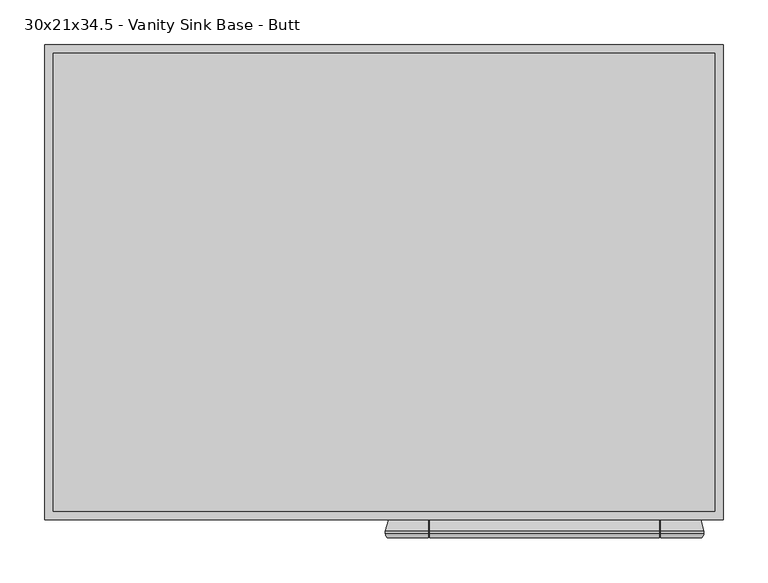
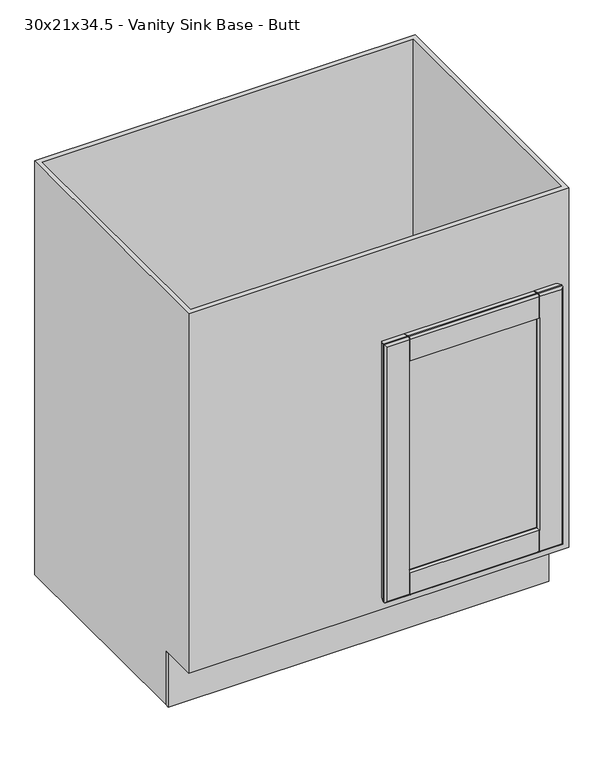
"""IFC4 building model written with IfcOpenShell, lengths in millimetres: furniture geometry, Cabinet-Base-Merillat-Double_Door-Marlin : 30x21x34.5 - Vanity Sink Base - Butt."""

from ifc_helpers import new_model, si_unit, frame, origin, origin_with_axes, place, context, project, spatial, polyline, circle_curve, ellipse_curve, outline, extrude, faceted_brep, source, transform, mapped, element, save
from ifc_brep_helpers import plane_surface, cylinder_surface, advanced_brep


def furniture_30x21x34_5_vanity_sink_base_butt_b45b5ea9(model_context):
    return source(origin(), model_context, "Body", "SolidModel", [
        advanced_brep(
        [(377.5127049, -625.4496, 685.8), (374.4162124, -629.92, 682.7035075), (374.4162124, -629.92, 142.7964925), (377.5127049, -625.4496, 139.7), (377.5127049, -622.681, 139.7), (377.5127049, -622.681, 685.8), (374.0075049, -609.6, 143.2052), (374.0075049, -609.6, 682.2948), (329.3115422, -609.6, 637.5988372), (329.3115422, -609.6, 187.9011628), (328.9414105, -610.39375, 188.2712945), (326.8602514, -614.85681, 190.3524535), (326.8602514, -614.85681, 635.1475465), (328.9414105, -610.39375, 637.2287055), (328.2600209, -617.0969093, 188.952684), (328.2600209, -617.0969093, 636.547316), (342.5877049, -617.347, 174.625), (342.5877049, -617.347, 650.875), (342.5877049, -622.173, 174.625), (342.5877049, -622.173, 650.875), (328.2600209, -622.4230907, 188.952684), (328.2600209, -622.4230907, 636.547316), (326.8602514, -624.66319, 190.3524535), (326.8602514, -624.66319, 635.1475465), (328.9414105, -629.12625, 188.2712945), (329.3086747, -629.9138508, 187.9040302), (329.3115422, -629.92, 637.5988372), (328.9414105, -629.12625, 637.2287055), (329.3086747, -629.92, 142.7964925), (329.3086747, -625.4496, 139.7), (23.4216974, -629.92, 142.7964925), (20.3252049, -625.4496, 139.7), (68.4894236, -625.4496, 139.7), (68.4894236, -629.92, 142.7964925), (327.7211747, -625.4496, 139.7), (327.7211747, -629.92, 142.7964925), (70.0769236, -629.92, 142.7964925), (70.0769236, -625.4496, 139.7), (329.3086747, -622.681, 139.7), (20.3252049, -622.681, 139.7), (68.4894236, -622.681, 139.7), (327.7211747, -622.681, 139.7), (70.0769236, -622.681, 139.7), (329.3086747, -609.6, 143.2052), (23.8304049, -609.6, 143.2052), (68.4894236, -609.6, 143.2052), (327.7211747, -609.6, 143.2052), (70.0769236, -609.6, 143.2052), (70.9776584, -614.85681, 190.3524535), (327.7211747, -610.39375, 188.2712945), (327.7211747, -609.6, 187.9011628), (70.0769236, -609.6, 187.9011628), (70.0769236, -610.39375, 188.2712945), (68.8964994, -610.39375, 188.2712945), (69.577889, -617.0969093, 188.952684), (55.2502049, -617.347, 174.625), (55.2502049, -622.173, 174.625), (69.577889, -622.4230907, 188.952684), (70.9776584, -624.66319, 190.3524535), (68.8964994, -629.12625, 188.2712945), (70.0769236, -629.12625, 188.2712945), (70.0769236, -629.92, 187.9011628), (327.7211747, -629.92, 187.9011628), (327.7211747, -629.12625, 188.2712945), (23.4216974, -629.92, 682.7035075), (20.3252049, -625.4496, 685.8), (20.3252049, -622.681, 685.8), (23.8304049, -609.6, 682.2948), (68.5263677, -609.6, 187.9011628), (68.5263677, -609.6, 637.5988372), (68.8964994, -610.39375, 637.2287055), (70.9776584, -614.85681, 635.1475465), (69.577889, -617.0969093, 636.547316), (55.2502049, -617.347, 650.875), (55.2502049, -622.173, 650.875), (69.577889, -622.4230907, 636.547316), (70.9776584, -624.66319, 635.1475465), (68.8964994, -629.12625, 637.2287055), (68.5263677, -629.92, 637.5988372), (68.5263677, -629.92, 187.9011628), (68.4894236, -629.92, 682.7035075), (68.4894236, -625.4496, 685.8), (329.3086747, -625.4496, 685.8), (329.3086747, -629.92, 682.7035075), (70.0769236, -625.4496, 685.8), (70.0769236, -629.92, 682.7035075), (327.7211747, -629.92, 682.7035075), (327.7211747, -625.4496, 685.8), (68.4894236, -622.681, 685.8), (329.3086747, -622.681, 685.8), (70.0769236, -622.681, 685.8), (327.7211747, -622.681, 685.8), (68.4894236, -609.6, 682.2948), (329.3086747, -609.6, 682.2948), (70.0769236, -609.6, 682.2948), (327.7211747, -609.6, 682.2948), (70.0769236, -609.6, 637.5988372), (327.7211747, -609.6, 637.5988372), (70.0769236, -610.39375, 637.2287055), (327.7211747, -610.39375, 637.2287055), (327.7211747, -629.12625, 637.2287055), (327.7211747, -629.92, 637.5988372), (70.0769236, -629.92, 637.5988372), (70.0769236, -629.12625, 637.2287055), (70.0769236, -610.39375, 681.6857412), (70.0769236, -622.7855037, 685.00625), (70.0769236, -625.4496, 685.00625), (70.0769236, -629.12625, 682.5526052), (68.4894236, -629.12625, 637.2287055), (68.4894236, -629.12625, 682.5526052), (68.4894236, -625.4496, 685.00625), (68.4894236, -622.7855037, 685.00625), (68.4894236, -610.39375, 681.6857412), (68.4894236, -610.39375, 637.2287055), (329.3086747, -610.39375, 637.2287055), (329.3086747, -610.39375, 681.6857412), (329.3086747, -622.7855037, 685.00625), (329.3086747, -625.4496, 685.00625), (329.3086747, -629.12625, 682.5526052), (329.3086747, -629.12625, 637.2287055), (327.7211747, -629.12625, 682.5526052), (327.7211747, -625.4496, 685.00625), (327.7211747, -622.7855037, 685.00625), (327.7211747, -610.39375, 681.6857412), (329.3086747, -629.12625, 188.2712945), (329.3086747, -629.12625, 142.9473948), (329.3086747, -625.4496, 140.49375), (329.3086747, -622.7855037, 140.49375), (329.3086747, -610.39375, 143.8142588), (329.3086747, -610.39375, 188.2712945), (327.7211747, -610.39375, 143.8142588), (327.7211747, -622.7855037, 140.49375), (327.7211747, -625.4496, 140.49375), (327.7211747, -629.12625, 142.9473948), (70.0769236, -629.12625, 142.9473948), (70.0769236, -625.4496, 140.49375), (70.0769236, -622.7855037, 140.49375), (70.0769236, -610.39375, 143.8142588), (68.4894236, -629.12625, 188.2712945), (68.4894236, -610.39375, 188.2712945), (68.4894236, -610.39375, 143.8142588), (68.4894236, -622.7855037, 140.49375), (68.4894236, -625.4496, 140.49375), (68.4894236, -629.12625, 142.9473948)],
        [
            (0, 1, ellipse_curve(frame((372.7375049, -625.4496, 681.0248), z_axis=(0.7071067811865475, 0.0, -0.7071067811865475), x_axis=(0.7071067811865474, 0.0, 0.7071067811865476)), 6.7531526, 4.7752)),
            (1, 2),
            (2, 3, ellipse_curve(frame((372.7375049, -625.4496, 144.4752), z_axis=(0.7071067811865475, 0.0, 0.7071067811865475), x_axis=(-0.7071067811865474, 0.0, 0.7071067811865476)), 6.7531526, 4.7752)),
            (3, 0),
            (3, 4),
            (4, 5),
            (5, 0),
            (4, 6),
            (6, 7),
            (7, 5),
            (8, 9),
            (9, 10),
            (10, 11),
            (11, 12),
            (12, 13),
            (13, 8),
            (11, 14, ellipse_curve(frame((328.2875049, -615.5223492, 188.9252), z_axis=(0.7071067811865475, 0.0, 0.7071067811865475), x_axis=(-0.7071067811865474, 0.0, 0.7071067811865476)), 2.2271035, 1.5748)),
            (14, 15),
            (15, 12, ellipse_curve(frame((328.2875049, -615.5223492, 636.5748), z_axis=(0.7071067811865475, 0.0, -0.7071067811865475), x_axis=(0.7071067811865474, 0.0, 0.7071067811865476)), 2.2271035, 1.5748)),
            (14, 16),
            (16, 17),
            (17, 15),
            (16, 18),
            (18, 19),
            (19, 17),
            (18, 20),
            (20, 21),
            (21, 19),
            (20, 22, ellipse_curve(frame((328.2875049, -623.9976508, 188.9252), z_axis=(0.7071067811865475, 0.0, 0.7071067811865475), x_axis=(-0.7071067811865474, 0.0, 0.7071067811865476)), 2.2271035, 1.5748)),
            (22, 23),
            (23, 21, ellipse_curve(frame((328.2875049, -623.9976508, 636.5748), z_axis=(0.7071067811865475, 0.0, -0.7071067811865475), x_axis=(0.7071067811865474, 0.0, 0.7071067811865476)), 2.2271035, 1.5748)),
            (22, 24),
            (24, 25),
            (25, 26),
            (26, 27),
            (27, 23),
            (2, 28),
            (28, 29, circle_curve(frame((329.3086747, -625.4496, 144.4752), z_axis=(1.0, 0.0, 0.0), x_axis=(0.0, 1.0, 0.0)), 4.7752)),
            (29, 3),
            (30, 31, ellipse_curve(frame((25.1004049, -625.4496, 144.4752), z_axis=(0.7071067811865475, 0.0, -0.7071067811865475), x_axis=(0.7071067811865476, 0.0, 0.7071067811865474)), 6.7531526, 4.7752)),
            (31, 32),
            (32, 33, circle_curve(frame((68.4894236, -625.4496, 144.4752), z_axis=(-1.0, 0.0, 0.0), x_axis=(0.0, 1.0, 0.0)), 4.7752)),
            (33, 30),
            (34, 35, circle_curve(frame((327.7211747, -625.4496, 144.4752), z_axis=(-1.0, 0.0, 0.0), x_axis=(0.0, 1.0, 0.0)), 4.7752)),
            (35, 36),
            (36, 37, circle_curve(frame((70.0769236, -625.4496, 144.4752), z_axis=(1.0, 0.0, 0.0), x_axis=(0.0, 1.0, 0.0)), 4.7752)),
            (37, 34),
            (29, 38),
            (38, 4),
            (31, 39),
            (39, 40),
            (40, 32),
            (41, 34),
            (37, 42),
            (42, 41),
            (38, 43),
            (43, 6),
            (39, 44),
            (44, 45),
            (45, 40),
            (46, 41),
            (42, 47),
            (47, 46),
            (48, 11),
            (10, 49),
            (49, 50),
            (50, 51),
            (51, 52),
            (52, 53),
            (53, 48),
            (48, 54, ellipse_curve(frame((69.5504049, -615.5223492, 188.9252), z_axis=(0.7071067811865475, 0.0, -0.7071067811865475), x_axis=(0.7071067811865476, 0.0, 0.7071067811865474)), 2.2271035, 1.5748)),
            (54, 14),
            (54, 55),
            (55, 16),
            (55, 56),
            (56, 18),
            (56, 57),
            (57, 20),
            (57, 58, ellipse_curve(frame((69.5504049, -623.9976508, 188.9252), z_axis=(0.7071067811865475, 0.0, -0.7071067811865475), x_axis=(0.7071067811865476, 0.0, 0.7071067811865474)), 2.2271035, 1.5748)),
            (58, 22),
            (58, 59),
            (59, 60),
            (60, 61),
            (61, 62),
            (62, 63),
            (63, 24),
            (30, 64),
            (64, 65, ellipse_curve(frame((25.1004049, -625.4496, 681.0248), z_axis=(-0.7071067811865475, 0.0, -0.7071067811865475), x_axis=(0.7071067811865474, 0.0, -0.7071067811865476)), 6.7531526, 4.7752)),
            (65, 31),
            (65, 66),
            (66, 39),
            (66, 67),
            (67, 44),
            (68, 69),
            (69, 70),
            (70, 71),
            (71, 48),
            (53, 68),
            (71, 72, ellipse_curve(frame((69.5504049, -615.5223492, 636.5748), z_axis=(-0.7071067811865475, 0.0, -0.7071067811865475), x_axis=(0.7071067811865474, 0.0, -0.7071067811865476)), 2.2271035, 1.5748)),
            (72, 54),
            (72, 73),
            (73, 55),
            (73, 74),
            (74, 56),
            (74, 75),
            (75, 57),
            (75, 76, ellipse_curve(frame((69.5504049, -623.9976508, 636.5748), z_axis=(-0.7071067811865475, 0.0, -0.7071067811865475), x_axis=(0.7071067811865474, 0.0, -0.7071067811865476)), 2.2271035, 1.5748)),
            (76, 58),
            (76, 77),
            (77, 78),
            (78, 79),
            (79, 59),
            (64, 80),
            (80, 81, circle_curve(frame((68.4894236, -625.4496, 681.0248), z_axis=(-1.0, 0.0, 0.0), x_axis=(0.0, 1.0, 0.0)), 4.7752)),
            (81, 65),
            (0, 82),
            (82, 83, circle_curve(frame((329.3086747, -625.4496, 681.0248), z_axis=(1.0, 0.0, 0.0), x_axis=(0.0, 1.0, 0.0)), 4.7752)),
            (83, 1),
            (84, 85, circle_curve(frame((70.0769236, -625.4496, 681.0248), z_axis=(1.0, 0.0, 0.0), x_axis=(0.0, 1.0, 0.0)), 4.7752)),
            (85, 86),
            (86, 87, circle_curve(frame((327.7211747, -625.4496, 681.0248), z_axis=(-1.0, 0.0, 0.0), x_axis=(0.0, 1.0, 0.0)), 4.7752)),
            (87, 84),
            (81, 88),
            (88, 66),
            (5, 89),
            (89, 82),
            (90, 84),
            (87, 91),
            (91, 90),
            (88, 92),
            (92, 67),
            (7, 93),
            (93, 89),
            (94, 90),
            (91, 95),
            (95, 94),
            (43, 9),
            (8, 93),
            (92, 69),
            (68, 45),
            (96, 94),
            (95, 97),
            (97, 96),
            (50, 46),
            (47, 51),
            (12, 71),
            (70, 98),
            (98, 96),
            (97, 99),
            (99, 13),
            (15, 72),
            (17, 73),
            (19, 74),
            (21, 75),
            (23, 76),
            (27, 100),
            (100, 101),
            (101, 102),
            (102, 103),
            (103, 77),
            (83, 26),
            (25, 28),
            (33, 79),
            (78, 80),
            (85, 102),
            (101, 86),
            (35, 62),
            (61, 36),
            (98, 104),
            (104, 105),
            (105, 106),
            (106, 107, circle_curve(frame((70.0769236, -625.4496, 681.0248), z_axis=(1.0, 0.0, 0.0), x_axis=(0.0, 0.0, 1.0)), 3.98145)),
            (107, 103),
            (78, 108),
            (108, 109),
            (109, 110, circle_curve(frame((68.4894236, -625.4496, 681.0248), z_axis=(-1.0, 0.0, 0.0), x_axis=(0.0, 0.0, 1.0)), 3.98145)),
            (110, 111),
            (111, 112),
            (112, 113),
            (113, 69),
            (77, 108),
            (107, 109),
            (106, 110),
            (105, 111),
            (104, 112),
            (70, 113),
            (8, 114),
            (114, 115),
            (115, 116),
            (116, 117),
            (117, 118, circle_curve(frame((329.3086747, -625.4496, 681.0248), z_axis=(1.0, 0.0, 0.0), x_axis=(0.0, 0.0, 1.0)), 3.98145)),
            (118, 119),
            (119, 26),
            (100, 120),
            (120, 121, circle_curve(frame((327.7211747, -625.4496, 681.0248), z_axis=(-1.0, 0.0, 0.0), x_axis=(0.0, 0.0, 1.0)), 3.98145)),
            (121, 122),
            (122, 123),
            (123, 99),
            (119, 27),
            (118, 120),
            (117, 121),
            (116, 122),
            (115, 123),
            (114, 13),
            (25, 124),
            (124, 125),
            (125, 126, circle_curve(frame((329.3086747, -625.4496, 144.4752), z_axis=(1.0, 0.0, 0.0), x_axis=(0.0, 0.0, 1.0)), 3.98145)),
            (126, 127),
            (127, 128),
            (128, 129),
            (129, 9),
            (49, 130),
            (130, 131),
            (131, 132),
            (132, 133, circle_curve(frame((327.7211747, -625.4496, 144.4752), z_axis=(-1.0, 0.0, 0.0), x_axis=(0.0, 0.0, 1.0)), 3.98145)),
            (133, 63),
            (129, 10),
            (128, 130),
            (127, 131),
            (126, 132),
            (125, 133),
            (124, 24),
            (60, 134),
            (134, 135, circle_curve(frame((70.0769236, -625.4496, 144.4752), z_axis=(1.0, 0.0, 0.0), x_axis=(0.0, 0.0, 1.0)), 3.98145)),
            (135, 136),
            (136, 137),
            (137, 52),
            (138, 79),
            (68, 139),
            (139, 140),
            (140, 141),
            (141, 142),
            (142, 143, circle_curve(frame((68.4894236, -625.4496, 144.4752), z_axis=(-1.0, 0.0, 0.0), x_axis=(0.0, 0.0, 1.0)), 3.98145)),
            (143, 138),
            (138, 59),
            (53, 139),
            (137, 140),
            (136, 141),
            (135, 142),
            (134, 143),
        ],
        [
            cylinder_surface(frame((372.7375049, -625.4496, 685.8), z_axis=(0.0, 0.0, 1.0), x_axis=(0.0, 1.0, 0.0)), 4.7752),
            plane_surface(frame((377.5127049, -625.4496, 685.8), z_axis=(1.0, 0.0, 0.0), x_axis=(0.0, 0.0, -1.0))),
            plane_surface(frame((377.5127049, -622.681, 685.8), z_axis=(0.9659229350723619, 0.25882983502910506, 0.0), x_axis=(0.0, 0.0, -1.0))),
            plane_surface(frame((329.3115422, -609.6, 637.5988372), z_axis=(-0.9063077870366099, 0.4226182617407856, 0.0), x_axis=(0.0, 0.0, -1.0))),
            cylinder_surface(frame((328.2875049, -615.5223492, 685.8), z_axis=(0.0, 0.0, 1.0000000000000002), x_axis=(-0.01745240643729364, -0.9998476951563912, 0.0)), 1.5748),
            plane_surface(frame((328.2600209, -617.0969093, 636.547316), z_axis=(-0.017452406437322144, -0.9998476951563906, 0.0), x_axis=(0.0, 0.0, -1.0))),
            plane_surface(frame((342.5877049, -617.347, 650.875), z_axis=(-1.0, 0.0, 0.0), x_axis=(0.0, 0.0, -1.0))),
            plane_surface(frame((342.5877049, -622.173, 650.875), z_axis=(-0.01745240643727848, 0.9998476951563914, 0.0), x_axis=(0.0, 0.0, -1.0))),
            cylinder_surface(frame((328.2875049, -623.9976508, 685.8), z_axis=(0.0, 0.0, 1.0000000000000002), x_axis=(-0.9063077870367326, -0.42261826174052236, 0.0)), 1.5748),
            plane_surface(frame((326.8602514, -624.66319, 635.1475465), z_axis=(-0.9063077870366333, -0.4226182617407352, 0.0), x_axis=(0.0, 0.0, -1.0))),
            cylinder_surface(frame((377.5127049, -625.4496, 144.4752), z_axis=(1.0, 0.0, 0.0), x_axis=(0.0, 1.0, 0.0)), 4.7752),
            plane_surface(frame((377.5127049, -625.4496, 139.7), z_axis=(0.0, 0.0, -1.0), x_axis=(-1.0, 0.0, 0.0))),
            plane_surface(frame((377.5127049, -622.681, 139.7), z_axis=(0.0, 0.25882983502910506, -0.9659229350723619), x_axis=(-1.0, 0.0, 0.0))),
            plane_surface(frame((329.3115422, -609.6, 187.9011628), z_axis=(0.0, 0.4226182617407856, 0.9063077870366099), x_axis=(-1.0, 0.0, 0.0))),
            cylinder_surface(frame((377.5127049, -615.5223492, 188.9252), z_axis=(1.0000000000000002, 0.0, 0.0), x_axis=(0.0, -0.9998476951563912, 0.01745240643729364)), 1.5748),
            plane_surface(frame((328.2600209, -617.0969093, 188.952684), z_axis=(0.0, -0.9998476951563906, 0.017452406437322144), x_axis=(-1.0, 0.0, 0.0))),
            plane_surface(frame((342.5877049, -617.347, 174.625), z_axis=(0.0, 0.0, 1.0), x_axis=(-1.0, 0.0, 0.0))),
            plane_surface(frame((342.5877049, -622.173, 174.625), z_axis=(0.0, 0.9998476951563914, 0.01745240643727848), x_axis=(-1.0, 0.0, 0.0))),
            cylinder_surface(frame((377.5127049, -623.9976508, 188.9252), z_axis=(1.0000000000000002, 0.0, 0.0), x_axis=(0.0, -0.42261826174052236, 0.9063077870367326)), 1.5748),
            plane_surface(frame((326.8602514, -624.66319, 190.3524535), z_axis=(0.0, -0.4226182617407352, 0.9063077870366333), x_axis=(-1.0, 0.0, 0.0))),
            cylinder_surface(frame((25.1004049, -625.4496, 139.7), z_axis=(0.0, 0.0, -1.0), x_axis=(0.0, 1.0, 0.0)), 4.7752),
            plane_surface(frame((20.3252049, -625.4496, 139.7), z_axis=(-1.0, 0.0, 0.0), x_axis=(0.0, 0.0, 1.0))),
            plane_surface(frame((20.3252049, -622.681, 139.7), z_axis=(-0.9659229350723619, 0.25882983502910506, 0.0), x_axis=(0.0, 0.0, 1.0))),
            plane_surface(frame((68.5263677, -609.6, 187.9011628), z_axis=(0.9063077870366099, 0.4226182617407856, 0.0), x_axis=(0.0, 0.0, 1.0))),
            cylinder_surface(frame((69.5504049, -615.5223492, 139.7), z_axis=(0.0, 0.0, -1.0000000000000002), x_axis=(0.01745240643729364, -0.9998476951563912, 0.0)), 1.5748),
            plane_surface(frame((69.577889, -617.0969093, 188.952684), z_axis=(0.017452406437322144, -0.9998476951563906, 0.0), x_axis=(0.0, 0.0, 1.0))),
            plane_surface(frame((55.2502049, -617.347, 174.625), z_axis=(1.0, 0.0, 0.0), x_axis=(0.0, 0.0, 1.0))),
            plane_surface(frame((55.2502049, -622.173, 174.625), z_axis=(0.01745240643727848, 0.9998476951563914, 0.0), x_axis=(0.0, 0.0, 1.0))),
            cylinder_surface(frame((69.5504049, -623.9976508, 139.7), z_axis=(0.0, 0.0, -1.0000000000000002), x_axis=(0.9063077870367326, -0.42261826174052236, 0.0)), 1.5748),
            plane_surface(frame((70.9776584, -624.66319, 190.3524535), z_axis=(0.9063077870366333, -0.4226182617407352, 0.0), x_axis=(0.0, 0.0, 1.0))),
            cylinder_surface(frame((20.3252049, -625.4496, 681.0248), z_axis=(-1.0, 0.0, 0.0), x_axis=(0.0, 1.0, 0.0)), 4.7752),
            plane_surface(frame((20.3252049, -625.4496, 685.8), z_axis=(0.0, 0.0, 1.0), x_axis=(1.0, 0.0, 0.0))),
            plane_surface(frame((20.3252049, -622.681, 685.8), z_axis=(0.0, 0.25882983502910506, 0.9659229350723619), x_axis=(1.0, 0.0, 0.0))),
            plane_surface(frame((23.8304049, -609.6, 682.2948), z_axis=(0.0, 1.0, 0.0), x_axis=(1.0, 0.0, 0.0))),
            plane_surface(frame((68.5263677, -609.6, 637.5988372), z_axis=(0.0, 0.4226182617407856, -0.9063077870366099), x_axis=(1.0, 0.0, 0.0))),
            cylinder_surface(frame((20.3252049, -615.5223492, 636.5748), z_axis=(-1.0000000000000002, 0.0, 0.0), x_axis=(0.0, -0.9998476951563912, -0.01745240643729364)), 1.5748),
            plane_surface(frame((69.577889, -617.0969093, 636.547316), z_axis=(0.0, -0.9998476951563906, -0.017452406437322144), x_axis=(1.0, 0.0, 0.0))),
            plane_surface(frame((55.2502049, -617.347, 650.875), z_axis=(0.0, 0.0, -1.0), x_axis=(1.0, 0.0, 0.0))),
            plane_surface(frame((55.2502049, -622.173, 650.875), z_axis=(0.0, 0.9998476951563914, -0.01745240643727848), x_axis=(1.0, 0.0, 0.0))),
            cylinder_surface(frame((20.3252049, -623.9976508, 636.5748), z_axis=(-1.0000000000000002, 0.0, 0.0), x_axis=(0.0, -0.42261826174052236, -0.9063077870367326)), 1.5748),
            plane_surface(frame((70.9776584, -624.66319, 635.1475465), z_axis=(0.0, -0.4226182617407352, -0.9063077870366333), x_axis=(1.0, 0.0, 0.0))),
            plane_surface(frame((68.5263677, -629.92, 637.5988372), z_axis=(0.0, -1.0, 0.0), x_axis=(1.0, 0.0, 0.0))),
            plane_surface(frame((70.0769236, -629.92, 637.5988372), z_axis=(-1.0, 0.0, 0.0), x_axis=(0.0, 0.906307787036771, -0.4226182617404399))),
            plane_surface(frame((68.4894236, -629.92, 637.5988372), z_axis=(1.0, 0.0, 0.0), x_axis=(0.0, -0.906307787036771, 0.4226182617404399))),
            plane_surface(frame((70.0769236, -629.92, 637.5988372), z_axis=(0.0, 0.4226182617404399, 0.906307787036771), x_axis=(-1.0, 0.0, 0.0))),
            plane_surface(frame((70.0769236, -629.12625, 637.2287055), z_axis=(0.0, -1.0, 0.0), x_axis=(-1.0, 0.0, 0.0))),
            cylinder_surface(frame((68.4894236, -625.4496, 681.0248), z_axis=(-1.0, 0.0, 0.0), x_axis=(0.0, 0.0, 1.0)), 3.98145),
            plane_surface(frame((70.0769236, -625.4496, 685.00625), z_axis=(0.0, 0.0, 1.0), x_axis=(-1.0, 0.0, 0.0))),
            plane_surface(frame((70.0769236, -622.7855037, 685.00625), z_axis=(0.0, 0.25882983502913415, 0.9659229350723542), x_axis=(-1.0, 0.0, 0.0))),
            plane_surface(frame((70.0769236, -610.39375, 681.6857412), z_axis=(0.0, 1.0, 0.0), x_axis=(-1.0, 0.0, 0.0))),
            plane_surface(frame((70.0769236, -610.39375, 637.2287055), z_axis=(0.0, -0.4226182617405111, 0.9063077870367379), x_axis=(-1.0, 0.0, 0.0))),
            plane_surface(frame((329.3086747, -629.92, 637.5988372), z_axis=(-1.0, 0.0, 0.0), x_axis=(0.0, 0.9063077870367783, -0.42261826174042444))),
            plane_surface(frame((327.7211747, -629.92, 637.5988372), z_axis=(1.0, 0.0, 0.0), x_axis=(0.0, -0.9063077870367783, 0.42261826174042444))),
            plane_surface(frame((329.3086747, -629.92, 637.5988372), z_axis=(0.0, 0.42261826174042444, 0.9063077870367783), x_axis=(-1.0, 0.0, 0.0))),
            plane_surface(frame((329.3086747, -629.12625, 637.2287055), z_axis=(0.0, -1.0, 0.0), x_axis=(-1.0, 0.0, 0.0))),
            cylinder_surface(frame((327.7211747, -625.4496, 681.0248), z_axis=(-1.0, 0.0, 0.0), x_axis=(0.0, 0.0, 1.0)), 3.98145),
            plane_surface(frame((329.3086747, -625.4496, 685.00625), z_axis=(0.0, 0.0, 1.0), x_axis=(-1.0, 0.0, 0.0))),
            plane_surface(frame((329.3086747, -622.7855037, 685.00625), z_axis=(0.0, 0.25882983502911566, 0.965922935072359), x_axis=(-1.0, 0.0, 0.0))),
            plane_surface(frame((329.3086747, -610.39375, 681.6857412), z_axis=(0.0, 1.0, 0.0), x_axis=(-1.0, 0.0, 0.0))),
            plane_surface(frame((329.3086747, -610.39375, 637.2287055), z_axis=(0.0, -0.42261826174056427, 0.9063077870367131), x_axis=(-1.0, 0.0, 0.0))),
            plane_surface(frame((329.3086747, -625.4496, 149.2504), z_axis=(-1.0, 0.0, 0.0), x_axis=(0.0, -1.0, 0.0))),
            plane_surface(frame((327.7211747, -625.4496, 149.2504), z_axis=(1.0, 0.0, 0.0), x_axis=(0.0, 1.0, 0.0))),
            plane_surface(frame((329.3086747, -609.6, 187.9011628), z_axis=(0.0, -0.42261826173999295, -0.9063077870369795), x_axis=(-1.0, 0.0, 0.0))),
            plane_surface(frame((329.3086747, -610.39375, 188.2712945), z_axis=(0.0, 1.0, 0.0), x_axis=(-1.0, 0.0, 0.0))),
            plane_surface(frame((329.3086747, -610.39375, 143.8142588), z_axis=(0.0, 0.2588298350290845, -0.9659229350723675), x_axis=(-1.0, 0.0, 0.0))),
            plane_surface(frame((329.3086747, -622.7855037, 140.49375), z_axis=(0.0, 0.0, -1.0), x_axis=(-1.0, 0.0, 0.0))),
            cylinder_surface(frame((327.7211747, -625.4496, 144.4752), z_axis=(-1.0, 0.0, 0.0), x_axis=(0.0, 0.0, 1.0)), 3.98145),
            plane_surface(frame((329.3086747, -629.12625, 142.9473948), z_axis=(0.0, -1.0, 0.0), x_axis=(-1.0, 0.0, 0.0))),
            plane_surface(frame((329.3086747, -629.12625, 188.2712945), z_axis=(0.0, 0.4226182617407698, -0.9063077870366172), x_axis=(-1.0, 0.0, 0.0))),
            plane_surface(frame((70.0769236, -629.12625, 188.2712945), z_axis=(-1.0, 0.0, 0.0), x_axis=(0.0, -0.906307787036583, -0.42261826174084305))),
            plane_surface(frame((68.4894236, -629.12625, 188.2712945), z_axis=(1.0, 0.0, 0.0), x_axis=(0.0, 0.906307787036583, 0.42261826174084305))),
            plane_surface(frame((70.0769236, -629.12625, 188.2712945), z_axis=(0.0, 0.42261826174084305, -0.906307787036583), x_axis=(-1.0, 0.0, 0.0))),
            plane_surface(frame((70.0769236, -609.6, 187.9011628), z_axis=(0.0, -0.42261826174073325, -0.9063077870366342), x_axis=(-1.0, 0.0, 0.0))),
            plane_surface(frame((70.0769236, -610.39375, 188.2712945), z_axis=(0.0, 1.0, 0.0), x_axis=(-1.0, 0.0, 0.0))),
            plane_surface(frame((70.0769236, -610.39375, 143.8142588), z_axis=(0.0, 0.2588298350290967, -0.9659229350723642), x_axis=(-1.0, 0.0, 0.0))),
            plane_surface(frame((70.0769236, -622.7855037, 140.49375), z_axis=(0.0, 0.0, -1.0), x_axis=(-1.0, 0.0, 0.0))),
            cylinder_surface(frame((68.4894236, -625.4496, 144.4752), z_axis=(-1.0, 0.0, 0.0), x_axis=(0.0, 0.0, 1.0)), 3.98145),
            plane_surface(frame((70.0769236, -629.12625, 142.9473948), z_axis=(0.0, -1.0, 0.0), x_axis=(-1.0, 0.0, 0.0))),
        ],
        [
            (0, [[1, 2, 3, 4]]),
            (1, [[-4, 5, 6, 7]]),
            (2, [[-6, 8, 9, 10]]),
            (3, [[11, 12, 13, 14, 15, 16]]),
            (4, [[-14, 17, 18, 19]]),
            (5, [[-18, 20, 21, 22]]),
            (6, [[-21, 23, 24, 25]]),
            (7, [[-24, 26, 27, 28]]),
            (8, [[-27, 29, 30, 31]]),
            (9, [[-30, 32, 33, 34, 35, 36]]),
            (10, [[-3, 37, 38, 39]]),
            (10, [[40, 41, 42, 43]]),
            (10, [[44, 45, 46, 47]]),
            (11, [[-5, -39, 48, 49]]),
            (11, [[50, 51, 52, -41]]),
            (11, [[53, -47, 54, 55]]),
            (12, [[-8, -49, 56, 57]]),
            (12, [[58, 59, 60, -51]]),
            (12, [[61, -55, 62, 63]]),
            (13, [[64, -13, 65, 66, 67, 68, 69, 70]]),
            (14, [[-17, -64, 71, 72]]),
            (15, [[-20, -72, 73, 74]]),
            (16, [[-23, -74, 75, 76]]),
            (17, [[-26, -76, 77, 78]]),
            (18, [[-29, -78, 79, 80]]),
            (19, [[-80, 81, 82, 83, 84, 85, 86, -32]]),
            (20, [[-40, 87, 88, 89]]),
            (21, [[-50, -89, 90, 91]]),
            (22, [[-58, -91, 92, 93]]),
            (23, [[94, 95, 96, 97, -70, 98]]),
            (24, [[-71, -97, 99, 100]]),
            (25, [[-73, -100, 101, 102]]),
            (26, [[-75, -102, 103, 104]]),
            (27, [[-77, -104, 105, 106]]),
            (28, [[-79, -106, 107, 108]]),
            (29, [[-108, 109, 110, 111, 112, -81]]),
            (30, [[-88, 113, 114, 115]]),
            (30, [[-1, 116, 117, 118]]),
            (30, [[119, 120, 121, 122]]),
            (31, [[-90, -115, 123, 124]]),
            (31, [[-7, 125, 126, -116]]),
            (31, [[127, -122, 128, 129]]),
            (32, [[-92, -124, 130, 131]]),
            (32, [[-10, 132, 133, -125]]),
            (32, [[134, -129, 135, 136]]),
            (33, [[-9, -57, 137, -11, 138, -132]]),
            (33, [[-93, -131, 139, -94, 140, -59]]),
            (33, [[141, -136, 142, 143]]),
            (33, [[144, -63, 145, -67]]),
            (34, [[146, -96, 147, 148, -143, 149, 150, -15]]),
            (35, [[-19, 151, -99, -146]]),
            (36, [[-22, 152, -101, -151]]),
            (37, [[-25, 153, -103, -152]]),
            (38, [[-28, 154, -105, -153]]),
            (39, [[-31, 155, -107, -154]]),
            (40, [[-155, -36, 156, 157, 158, 159, 160, -109]]),
            (41, [[-2, -118, 161, -34, 162, -37]]),
            (41, [[-87, -43, 163, -111, 164, -113]]),
            (41, [[165, -158, 166, -120]]),
            (41, [[167, -84, 168, -45]]),
            (42, [[169, 170, 171, 172, 173, -159, -165, -119, -127, -134, -141, -148]]),
            (43, [[174, 175, 176, 177, 178, 179, 180, -139, -130, -123, -114, -164]]),
            (44, [[-174, -110, 181]]),
            (45, [[-173, 182, -175, -181, -160]]),
            (46, [[-172, 183, -176, -182]]),
            (47, [[-171, 184, -177, -183]]),
            (48, [[-170, 185, -178, -184]]),
            (49, [[-169, -147, 186, -179, -185]]),
            (50, [[-180, -186, -95]]),
            (51, [[187, 188, 189, 190, 191, 192, 193, -161, -117, -126, -133, -138]]),
            (52, [[194, 195, 196, 197, 198, -149, -142, -135, -128, -121, -166, -157]]),
            (53, [[-193, 199, -35]]),
            (54, [[-192, 200, -194, -156, -199]]),
            (55, [[-191, 201, -195, -200]]),
            (56, [[-190, 202, -196, -201]]),
            (57, [[-189, 203, -197, -202]]),
            (58, [[-188, 204, -150, -198, -203]]),
            (59, [[-187, -16, -204]]),
            (60, [[205, 206, 207, 208, 209, 210, 211, -137, -56, -48, -38, -162]]),
            (61, [[212, 213, 214, 215, 216, -85, -167, -44, -53, -61, -144, -66]]),
            (62, [[-211, 217, -12]]),
            (63, [[-210, 218, -212, -65, -217]]),
            (64, [[-209, 219, -213, -218]]),
            (65, [[-208, 220, -214, -219]]),
            (66, [[-207, 221, -215, -220]]),
            (67, [[-206, 222, -86, -216, -221]]),
            (68, [[-205, -33, -222]]),
            (69, [[223, 224, 225, 226, 227, -68, -145, -62, -54, -46, -168, -83]]),
            (70, [[228, -163, -42, -52, -60, -140, 229, 230, 231, 232, 233, 234]]),
            (71, [[-228, 235, -112]]),
            (72, [[-229, -98, 236]]),
            (73, [[-227, 237, -230, -236, -69]]),
            (74, [[-226, 238, -231, -237]]),
            (75, [[-225, 239, -232, -238]]),
            (76, [[-224, 240, -233, -239]]),
            (77, [[-223, -82, -235, -234, -240]]),
        ],
    ),
        extrude(outline(polyline([(55.2502049, -622.173), (55.2502049, -617.347), (342.5877049, -617.347), (342.5877049, -622.173), (55.2502049, -622.173)])), frame((0.0, 0.0, 174.625), z_axis=(0.0, 0.0, 1.0), x_axis=(1.0, 0.0, 0.0)), (0.0, 0.0, 1.0), 476.25),
        faceted_brep([(399.7377049, -76.2, 0.0), (399.7377049, -529.43125, 0.0), (390.2127049, -529.43125, 0.0), (390.2127049, -85.725, 0.0), (-352.7372951, -85.725, 0.0), (-352.7372951, -529.43125, 0.0), (-362.2622951, -529.43125, 0.0), (-362.2622951, -76.2, 0.0), (-362.2622951, -76.2, 876.3), (399.7377049, -76.2, 876.3), (-362.2622951, -529.43125, 114.3), (-362.2622951, -609.6, 114.3), (-362.2622951, -609.6, 876.3), (399.7377049, -609.6, 876.3), (399.7377049, -609.6, 114.3), (399.7377049, -529.43125, 114.3), (390.2127049, -529.43125, 114.3), (390.2127049, -85.725, 114.3), (390.2127049, -600.075, 876.3), (390.2127049, -85.725, 876.3), (390.2127049, -85.725, 123.825), (390.2127049, -600.075, 123.825), (-352.7372951, -85.725, 114.3), (-352.7372951, -529.43125, 114.3), (-352.7372951, -85.725, 876.3), (-352.7372951, -600.075, 876.3), (-352.7372951, -600.075, 123.825), (-352.7372951, -85.725, 123.825)], [[[0, 1, 2, 3, 4, 5, 6, 7]], [[0, 7, 8, 9]], [[7, 6, 10, 11, 12, 8]], [[1, 0, 9, 13, 14, 15]], [[3, 2, 16, 17]], [[18, 19, 20, 21]], [[5, 4, 22, 23]], [[24, 25, 26, 27]], [[4, 3, 17, 22]], [[19, 24, 27, 20]], [[9, 8, 12, 13], [19, 18, 25, 24]], [[14, 11, 10, 23, 22, 17, 16, 15]], [[13, 12, 11, 14]], [[25, 18, 21, 26]], [[6, 5, 23, 10]], [[2, 1, 15, 16]], [[21, 20, 27, 26]]]),
        extrude(outline(polyline([(399.7377049, -529.43125), (399.7377049, -538.95625), (-362.2622951, -538.95625), (-362.2622951, -529.43125), (399.7377049, -529.43125)])), origin_with_axes(), (0.0, 0.0, 1.0), 114.3),
    ])


if __name__ == "__main__":
    model = new_model("IFC4")
    model_context = context("Model", 3, world=origin())
    ifc_project = project(units=[si_unit("LENGTHUNIT", "METRE", prefix="MILLI")], contexts=[model_context])
    site = spatial("IfcSite", under=ifc_project)
    building = spatial("IfcBuilding", under=site)
    placement = place(None, origin())
    furniture_30x21x34_5_vanity_sink_base_butt_shape = furniture_30x21x34_5_vanity_sink_base_butt_b45b5ea9(model_context)
    element("IfcFurniture", 1, ObjectType="Cabinet-Base-Merillat-Double_Door-Marlin : 30x21x34.5 - Vanity Sink Base - Butt", at=placement, inside=building, context=model_context, shape_type="MappedRepresentation", body=[
        mapped(furniture_30x21x34_5_vanity_sink_base_butt_shape, transform((0.0, 0.0, 0.0), x_axis=(1.0, 0.0, 0.0), y_axis=(0.0, 1.0, 0.0), z_axis=(0.0, 0.0, 1.0))),
    ])
    save(model, "model.ifc")

# Revit data of these elements
# Type "Cabinet-Base-Merillat-Double_Door-Marlin : 30x21x34.5 - Vanity Sink Base - Butt"
#   URL = "http://www.merillat.com"
#   Toe Kick Note = "Toe Kick Covering is not included. To be purchased Separately."
#   Product Line = "Express"
#   Product Page URL = "http://www.merillat.com//our-products/rooms/bathroom"
#   Product Group = "Vanity Cabinet"
#   Product Documentation Link = "http://merillatbusiness.com/customer-resources/product-line-resources/merillat-classic/"
#   Model = "VSB3035B"
#   Manufacturer = "Merillat"
#   Finish = "Wood"
#   Description = "Vanity Sink Base Double Door"
#   Construction Type = "Deep Sink Base"
#   Cabinet Construction Note = "No shelf, cabinets w/ a \"B\" suffix have BUTT doors without a center frame stile,  VSB39, VSB42. VSB3935 and VSB4235 have a double door with a frame center stile, All cabinets have one full-width drawer front except VSB42 and VSB4235 which have two drawer fronts"
#   Assembly Code = "C1030410"
#   Toe Kick Height = 0' - 4 1/2"
#   Toe Kick Depth = 0' - 2 25/32"
#   Top and Bottom Spacing = 0' - 1"
#   Side Spacing = 0' - 0 7/8"
#   Cabinet Shell = 0' - 0 3/8"
#   Door Spacing = 0' - 0 1/8"
#   Depth = 1' - 9"
#   Height = 2' - 10 1/2"
#   Width = 2' - 6"
#   Cabinet Drawer Width = 2' - 4 1/4"
#   Cabinet Drawer Height = 0' - 5 1/2"
#   Cabinet Drawer 2 Drawer Width = 1' - 2 1/16"
#   Cabinet Door Width = 1' - 2 1/16"
#   Cabinet Door Height = 1' - 9 1/2"
#   COBie.Type = no
#   Two Drawer = no
#   Elevation Swing Line = yes
#   Partial Overlay = yes
#   One Drawer = yes
#   Full Overlay = no
#   Butt Option = yes
#   Toe Kick Material = Wood - Merillat - Raw Particle Board
#   Door Drawer Material = Wood - Merillat - Pecan(1)
#   Cabinet Material = Wood - Merillat - Pecan(1)
#   Cabinet Drawer Style 2 Drawer = element 819256
#   Cabinet Drawer Style = element 819255
#   Cabinet Door Style = element 819254
# Element 1 (IfcFurniture, "Cabinet-Base-Merillat-Double_Door-Marlin : 30x21x34.5 - Vanity Sink Base - Butt")
#   Materials on its faces: "Wood - Merillat - Pecan(1)", "Wood - Merillat - Raw Particle Board"
# Materials
#   "Wood - Merillat - Raw Particle Board": class "Plastic", colour RGB 80 80 80, transparency 0, Description = "Plastic Laminate - Navy", Cost = 0
#   "Wood - Merillat - Pecan(1)": class "Wood", colour RGB 108 67 43, transparency 0, Cost = 0
